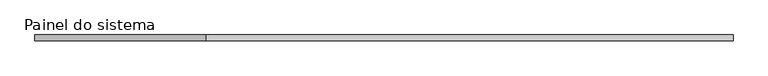
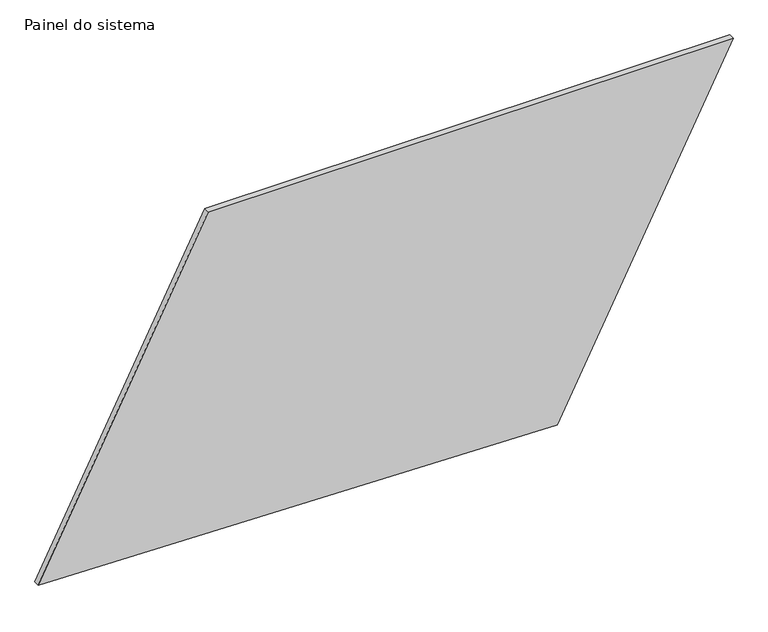
"""IFC4 building model written with IfcOpenShell, lengths in millimetres: plate geometry, Painel do sistema : Envidraçado."""

from ifc_helpers import new_model, si_unit, frame, origin, place, context, project, spatial, polyline, outline, extrude, source, transform, mapped, element, save


def painel_do_sistema_968a6b48(model_context):
    return source(origin(), model_context, "Body", "SweptSolid", [
        extrude(outline(polyline([(53.1539046, -1529.4256769), (0.0, 754.6859571), (1530.3339013, 1529.4256769), (1530.3339013, -781.5954055), (53.1539046, -1529.4256769)])), frame((0.0, 24.5, 0.0), z_axis=(0.0, 1.0, 0.0), x_axis=(0.0, 0.0, 1.0)), (0.0, 0.0, 1.0), 25.0),
    ])


if __name__ == "__main__":
    model = new_model("IFC4")
    model_context = context("Model", 3, world=origin())
    ifc_project = project(units=[si_unit("LENGTHUNIT", "METRE", prefix="MILLI")], contexts=[model_context])
    site = spatial("IfcSite", under=ifc_project)
    building = spatial("IfcBuilding", under=site)
    placement = place(None, origin())
    painel_do_sistema_shape = painel_do_sistema_968a6b48(model_context)
    element("IfcPlate", 1, ObjectType="Painel do sistema : Envidraçado", at=placement, inside=building, context=model_context, shape_type="MappedRepresentation", body=[
        mapped(painel_do_sistema_shape, transform((0.0, 0.0, 0.0), x_axis=(1.0, 0.0, 0.0), y_axis=(0.0, 1.0, 0.0), z_axis=(0.0, 0.0, 1.0))),
    ])
    save(model, "model.ifc")

# Revit data of these elements
# Type "Painel do sistema : Envidraçado"
#   Construction Type Id = "GSP4R"
#   Analytic Construction = "Vidraça única Pilkington 1/8 pol"
#   Visual Light Transmittance = 0.9
#   Solar Heat Gain Coefficient = 0.86
#   Heat Transfer Coefficient (U) = 6.7069 W/(m²·K)
# Element 1 (IfcPlate, "Painel do sistema : Envidraçado")
#   Materials on its faces: "Vidro"
# Materials
#   "Vidro": class "Vidro", colour RGB 0 128 192, transparency 0.9, Description = "Vidro de sílica", Cost = 0
